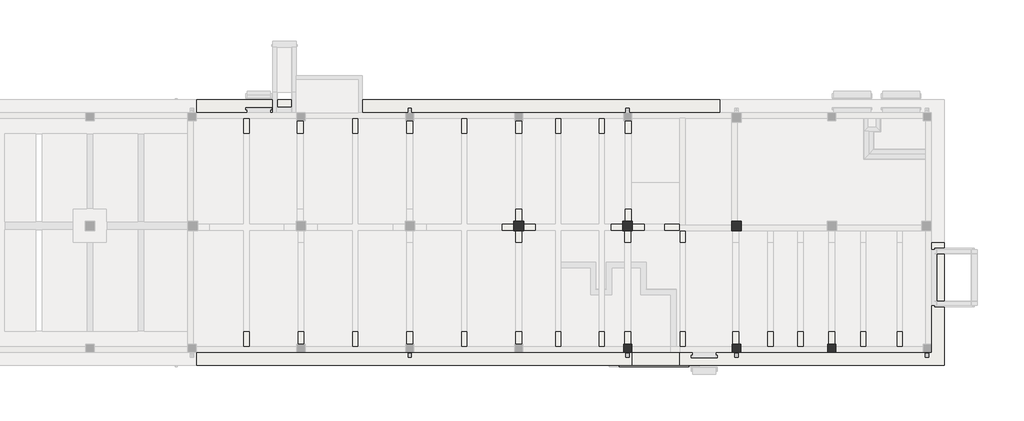
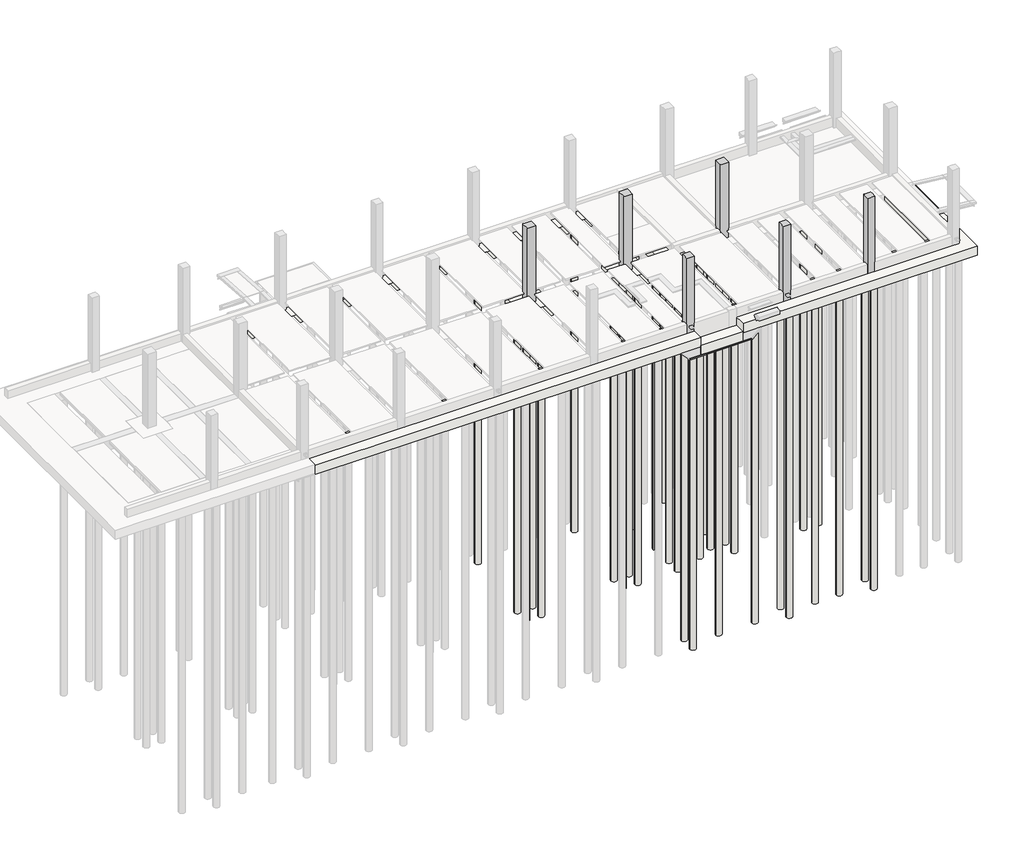
# One storey, part 5 of 7: 42 slabs, 6 columns.
# Revit data of these elements (continued)
# Elements 14, 15, 16, 17, 18, 19, 20, 21, 33, 34, 35, 36, 37, 38, 39, 40, 41, 42, 43, 44, 45, 46, 47, 48 (IfcSlab, "PILE : H_FL_AR S19_Pile_D500_L26.8")
#   Structural Material = Concrete_f'c=28MPa(Cylender)
#   Phase Created = New Construction
#   Materials on its faces: "Concrete_f'c=28MPa(Cylender)"
# Elements 22, 23, 24, 25, 26, 27, 28, 29 (IfcSlab, "PILE : H_FL_AR S19_Pile_D500_L26.6")
#   Structural Material = Concrete_f'c=28MPa(Cylender)
#   Phase Created = New Construction
#   Materials on its faces: "Concrete_f'c=28MPa(Cylender)"
# Elements 30, 31, 32 (IfcSlab, "PILE : H_FL_AR S19_Pile_D500_L26.1")
#   Structural Material = Concrete_f'c=28MPa(Cylender)
#   Phase Created = New Construction
#   Materials on its faces: "Concrete_f'c=28MPa(Cylender)"
# Materials
#   "Concrete_f'c=28MPa(Cylender)": class "Concrete", colour RGB 176 176 176, transparency 0, Description = "Reinf. Conc.", Cost = 0, Image = Concrete.Cast-In-Place.Flat.Polished.Grey.jpg
#   "Concrete_f'c=14MPa(Cylender)": class "Concrete", colour RGB 177 177 177, transparency 0, Description = "Reinf. Conc.", Cost = 0
